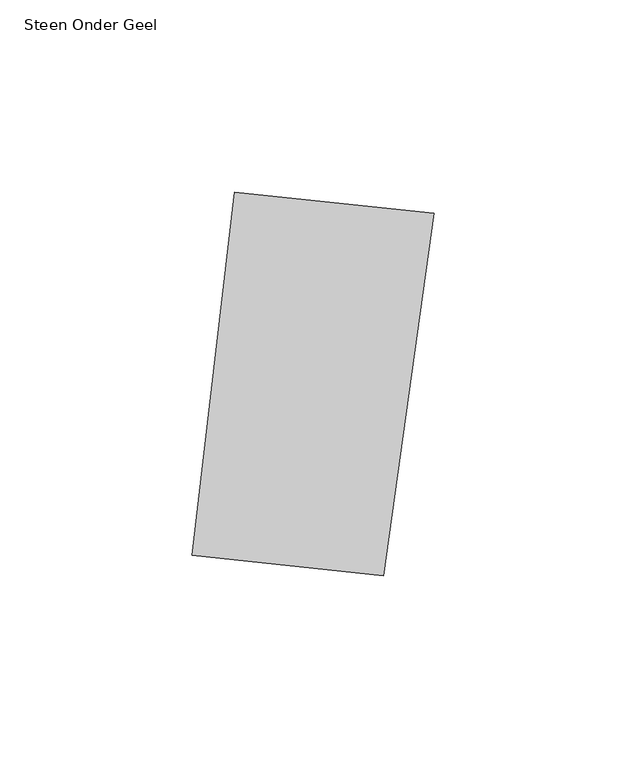
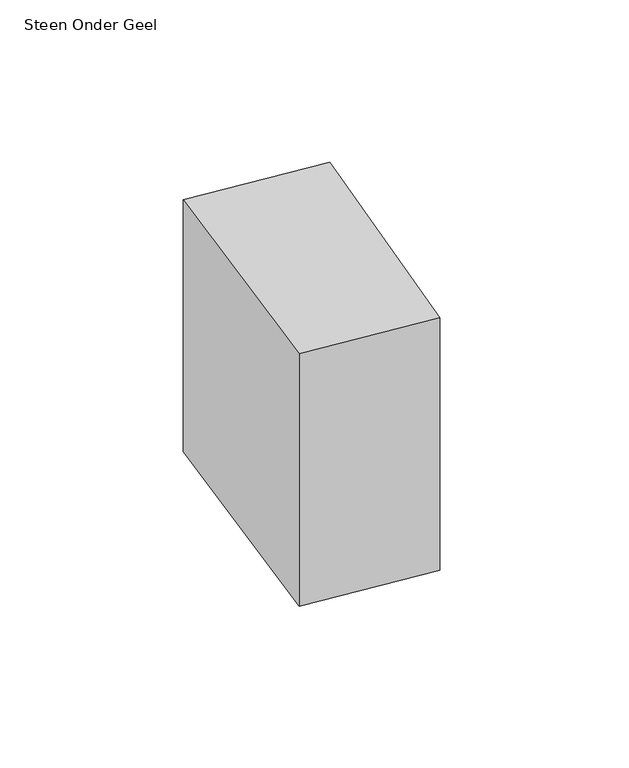
"""IFC4 building model written with IfcOpenShell, lengths in millimetres: proxy geometry, 00_GMA_steen_versie_4 : Steen Onder Geel."""

import ifcopenshell
import ifcopenshell.guid

model = None  # the IFC model being written
_history = None  # IfcOwnerHistory: only IFC2X3 demands one
_inside = {}  # id of a spatial element -> (the spatial element, [elements in it])
_under = {}  # id of a project, library or spatial element -> (it, [spatial elements below it])
_declared = {}  # id of a project -> (the project, [libraries it declares])
_typed = {}  # id of a type object -> (the type object, [elements of that type])
_made_of = {}  # id of a material, layer set ... -> (it, [elements and type objects made of it])


def new_model(schema):
    """Start an empty IFC model of exactly this schema.

    Asked for "IFC4X3", IfcOpenShell would pick the latest addendum, in which some entities
    have other attributes; the version numbers below select the first issue.
    IFC2X3 requires an IfcOwnerHistory on every rooted entity: one is made here for all.
    """
    global model, _history
    if schema == "IFC4X3":
        model = ifcopenshell.file(schema_version=(4, 3, 0, 0))
    else:
        model = ifcopenshell.file(schema=schema)
    _inside.clear()
    _under.clear()
    _declared.clear()
    _typed.clear()
    _made_of.clear()
    _history = None
    if model.schema == "IFC2X3":
        org = make("IfcOrganization", Name="unknown")
        user = make(
            "IfcPersonAndOrganization",
            ThePerson=make("IfcPerson", FamilyName="unknown"),
            TheOrganization=org,
        )
        app = make(
            "IfcApplication",
            ApplicationDeveloper=org,
            Version="unknown",
            ApplicationFullName="unknown",
            ApplicationIdentifier="unknown",
        )
        _history = make(
            "IfcOwnerHistory",
            OwningUser=user,
            OwningApplication=app,
            ChangeAction="ADDED",
            CreationDate=0,
        )
    return model


def make(cls, **values):
    """One entity of the class cls with the attributes given. An attribute that is None is left unset."""
    return model.create_entity(
        cls, **{name: value for name, value in values.items() if value is not None}
    )


def rooted(cls, **values):
    """An entity with a GlobalId (a new one), such as an element, a storey or a relation."""
    return make(cls, GlobalId=ifcopenshell.guid.new(), OwnerHistory=_history, **values)


def si_unit(unit_type, name, prefix=None):
    """IfcSIUnit, for example si_unit("LENGTHUNIT", "METRE", prefix="MILLI")."""
    return make("IfcSIUnit", UnitType=unit_type, Prefix=prefix, Name=name)


def assignment(units):
    """IfcUnitAssignment: the units of a project."""
    return None if units is None else make("IfcUnitAssignment", Units=units)


def point(xyz):
    """IfcCartesianPoint."""
    return None if xyz is None else make("IfcCartesianPoint", Coordinates=xyz)


def direction(xyz):
    """IfcDirection."""
    return None if xyz is None else make("IfcDirection", DirectionRatios=xyz)


def frame(location, z_axis=None, x_axis=None):
    """IfcAxis2Placement3D, a coordinate frame: its origin and axes. An axis left out is left unset."""
    return make(
        "IfcAxis2Placement3D",
        Location=point(location),
        Axis=direction(z_axis),
        RefDirection=direction(x_axis),
    )


def origin():
    """The frame at (0, 0, 0) with its axes left unset."""
    return frame((0.0, 0.0, 0.0))


def origin_with_axes():
    """The frame at (0, 0, 0) with the z axis (0, 0, 1) and the x axis (1, 0, 0) written out."""
    return frame((0.0, 0.0, 0.0), z_axis=(0.0, 0.0, 1.0), x_axis=(1.0, 0.0, 0.0))


def place(relative_to, where):
    """IfcLocalPlacement: puts the frame where relative to a parent placement (None: the world)."""
    return make(
        "IfcLocalPlacement", PlacementRelTo=relative_to, RelativePlacement=where
    )


def context(
    kind, dimensions, precision=None, world=None, true_north=None, identifier=None
):
    """IfcGeometricRepresentationContext, for example the 3D "Model" context."""
    return make(
        "IfcGeometricRepresentationContext",
        ContextIdentifier=identifier,
        ContextType=kind,
        CoordinateSpaceDimension=dimensions,
        Precision=precision,
        WorldCoordinateSystem=world,
        TrueNorth=true_north,
    )


def project(units=None, contexts=None):
    """IfcProject with its units and contexts."""
    return rooted(
        "IfcProject",
        Name="project",
        RepresentationContexts=contexts,
        UnitsInContext=assignment(units),
    )


def spatial(cls, under=None, at=None, **own):
    """A site, building, storey or space (cls), placed at a placement, below another one or the project."""
    s = rooted(cls, ObjectPlacement=at, **own)
    if under is not None:
        _under.setdefault(under.id(), (under, []))[1].append(s)
    return s


def polyline(points):
    """IfcPolyline through the points."""
    return make("IfcPolyline", Points=[point(p) for p in points])


def outline(outer, holes=None, kind="AREA"):
    """IfcArbitraryClosedProfileDef: a profile drawn as a closed curve; with holes, ...WithVoids."""
    if holes is None:
        return make("IfcArbitraryClosedProfileDef", ProfileType=kind, OuterCurve=outer)
    return make(
        "IfcArbitraryProfileDefWithVoids",
        ProfileType=kind,
        OuterCurve=outer,
        InnerCurves=holes,
    )


def extrude(swept, where, along, depth):
    """IfcExtrudedAreaSolid: the profile swept, set in the frame where, extruded along a direction by depth."""
    return make(
        "IfcExtrudedAreaSolid",
        SweptArea=swept,
        Position=where,
        ExtrudedDirection=direction(along),
        Depth=depth,
    )


def shape(context_of_items, identifier, shape_type, items):
    """IfcShapeRepresentation: the items that make up one representation, for example the "Body"."""
    return make(
        "IfcShapeRepresentation",
        ContextOfItems=context_of_items,
        RepresentationIdentifier=identifier,
        RepresentationType=shape_type,
        Items=items,
    )


def source(mapping_origin, context_of_items, identifier, shape_type, items):
    """IfcRepresentationMap: a shape defined once, which mapped items show again and again."""
    return make(
        "IfcRepresentationMap",
        MappingOrigin=mapping_origin,
        MappedRepresentation=shape(context_of_items, identifier, shape_type, items),
    )


def transform(
    local_origin,
    x_axis=None,
    y_axis=None,
    z_axis=None,
    scale=None,
    scale2=None,
    scale3=None,
    uniform=True,
):
    """IfcCartesianTransformationOperator3D, or its non-uniform kind. x_axis, y_axis, z_axis: its Axis1, 2, 3."""
    if uniform:
        return make(
            "IfcCartesianTransformationOperator3D",
            Axis1=direction(x_axis),
            Axis2=direction(y_axis),
            LocalOrigin=point(local_origin),
            Scale=scale,
            Axis3=direction(z_axis),
        )
    return make(
        "IfcCartesianTransformationOperator3DnonUniform",
        Axis1=direction(x_axis),
        Axis2=direction(y_axis),
        LocalOrigin=point(local_origin),
        Scale=scale,
        Axis3=direction(z_axis),
        Scale2=scale2,
        Scale3=scale3,
    )


def mapped(mapping_source, mapping_target):
    """IfcMappedItem: shows the shape of a source again, moved by a transform."""
    return make(
        "IfcMappedItem", MappingSource=mapping_source, MappingTarget=mapping_target
    )


def made_of(thing, what):
    """Note that an element or type object is made of a material, layer set ...; save() writes the relation."""
    if what is not None:
        _made_of.setdefault(what.id(), (what, []))[1].append(thing)
    return thing


def element(
    cls,
    number,
    at=None,
    inside=None,
    cuts=None,
    type_object=None,
    material=None,
    context=None,
    identifier="Body",
    shape_type=None,
    held_by="IfcProductDefinitionShape",
    body=None,
    shapes=None,
    **own,
):
    """One element of the class cls, such as IfcWall. Its Tag is "e" and its number.

    at: its placement. inside: the storey or other place that contains it. cuts: it is an
    opening in that element (IfcRelVoidsElement). A single representation is given by context,
    identifier, shape_type and body (its items); several are given by shapes. held_by: the class
    of the entity that holds the representations. save() writes the other relations.
    """
    e = rooted(cls, Tag="e%d" % number, ObjectPlacement=at, **own)
    if body is not None:
        shapes = [shape(context, identifier, shape_type, body)]
    if shapes is not None:
        e.Representation = make(held_by, Representations=shapes)
    if inside is not None:
        _inside.setdefault(inside.id(), (inside, []))[1].append(e)
    if cuts is not None:
        rooted(
            "IfcRelVoidsElement", RelatingBuildingElement=cuts, RelatedOpeningElement=e
        )
    if type_object is not None:
        _typed.setdefault(type_object.id(), (type_object, []))[1].append(e)
    return made_of(e, material)


def aggregate(whole, parts):
    """IfcRelAggregates: a whole, such as a stair, and the parts it consists of."""
    return rooted("IfcRelAggregates", RelatingObject=whole, RelatedObjects=parts)


def save(model, path):
    """Write the relations noted so far, then the file.

    IfcRelAggregates (storeys below a building ...), IfcRelContainedInSpatialStructure (elements
    in a storey), IfcRelDefinesByType, IfcRelAssociatesMaterial and IfcRelDeclares: one each for
    every whole, place, type object, material and project.
    """
    for whole, parts in _under.values():
        aggregate(whole, parts)
    for where, things in _inside.values():
        rooted(
            "IfcRelContainedInSpatialStructure",
            RelatedElements=things,
            RelatingStructure=where,
        )
    for kind, things in _typed.values():
        rooted("IfcRelDefinesByType", RelatedObjects=things, RelatingType=kind)
    for what, things in _made_of.values():
        rooted("IfcRelAssociatesMaterial", RelatedObjects=things, RelatingMaterial=what)
    for by, libraries in _declared.values():
        rooted("IfcRelDeclares", RelatingContext=by, RelatedDefinitions=libraries)
    model.write(path)


def steen_onder_geel_1e791dec(model_context):
    return source(origin(), model_context, "Body", "SweptSolid", [
        extrude(outline(polyline([(106.7895948, 113.717828), (93.6822742, 19.5705172), (43.9577045, 24.8114308), (54.9652378, 119.1779756), (106.7895948, 113.717828)])), origin_with_axes(), (0.0, 0.0, 1.0), 100.0),
    ])


if __name__ == "__main__":
    model = new_model("IFC4")
    model_context = context("Model", 3, world=origin())
    ifc_project = project(units=[si_unit("LENGTHUNIT", "METRE", prefix="MILLI")], contexts=[model_context])
    site = spatial("IfcSite", under=ifc_project)
    building = spatial("IfcBuilding", under=site)
    placement = place(None, origin())
    steen_onder_geel_shape = steen_onder_geel_1e791dec(model_context)
    element("IfcBuildingElementProxy", 1, Name="00_GMA_steen_versie_4 : Steen Onder Geel", ObjectType="00_GMA_steen_versie_4 : Steen Onder Geel", at=placement, inside=building, context=model_context, shape_type="MappedRepresentation", body=[
        mapped(steen_onder_geel_shape, transform((0.0, 0.0, 0.0), x_axis=(1.0, 0.0, 0.0), y_axis=(0.0, 1.0, 0.0), z_axis=(0.0, 0.0, 1.0))),
    ])
    save(model, "model.ifc")

# Revit data of these elements
# Type "00_GMA_steen_versie_4 : Steen Onder Geel"
#   StootVoegHalfBoven [instance default] = 5 mm
#   StootVoegHalf [instance default] = 5 mm
#   StootVoegBreedteOnder = 10 mm
#   StootVoegBreedteBoven = 10 mm
#   Steendikte = 100 mm
#   LintVoegOnderHalf = 0 mm
#   LintVoegOnder = 0 mm
#   LintVoegBovenHalf = 5 mm
#   LintVoegBoven = 10 mm
#   materiaal = 21_steen_geel
#   MateriaalVoeg = none
#   Default Elevation = 0
# Element 1 (IfcBuildingElementProxy, "00_GMA_steen_versie_4 : Steen Onder Geel")
#   Materials on its faces: "21_steen_geel"
# Materials
#   "21_steen_geel": class "Unassigned", colour RGB 202 202 0, transparency 0, Cost = 0
